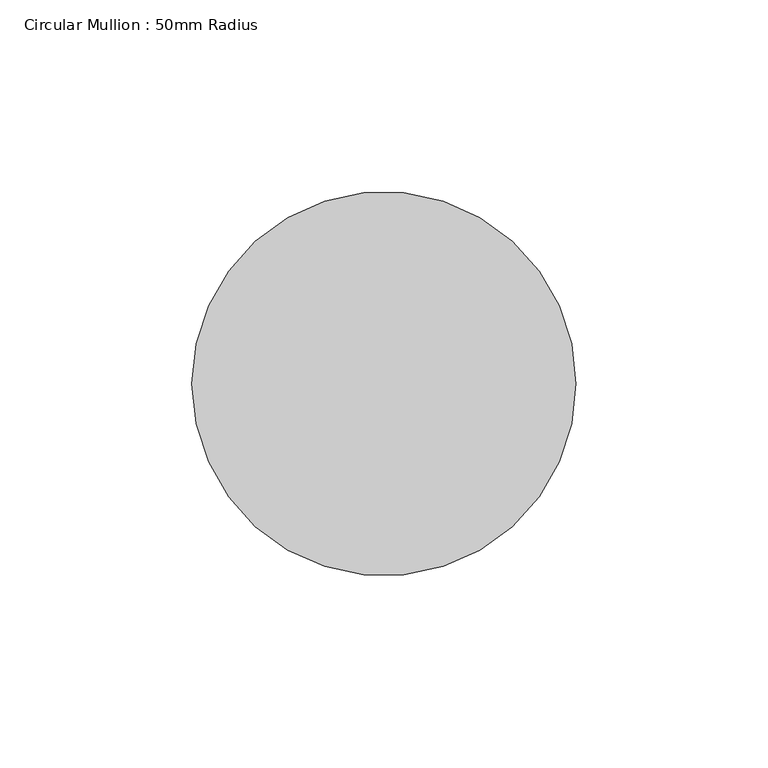
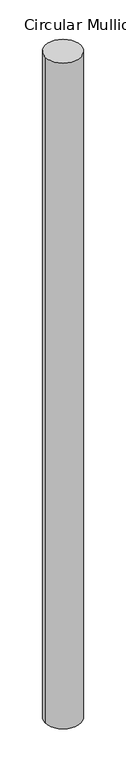
"""IFC4 building model written with IfcOpenShell, lengths in millimetres: member geometry, Circular Mullion : 50mm Radius."""

from ifc_helpers import new_model, si_unit, point, frame, frame_2d, origin, place, context, project, spatial, circle_curve, trimmed, segment, composite_curve, outline, extrude, source, transform, mapped, element, save


def circular_mullion_50mm_radius_29af998c(model_context):
    return source(origin(), model_context, "Body", "SweptSolid", [
        extrude(outline(composite_curve([segment(trimmed(circle_curve(frame_2d((-50.0, 0.0)), 50.0), [point((0.0, 0.0))], [point((-100.0, 0.0))], False, "CARTESIAN"), True, "CONTINUOUS"), segment(trimmed(circle_curve(frame_2d((-50.0, 0.0)), 50.0), [point((-100.0, 0.0))], [point((0.0, 0.0))], False, "CARTESIAN"), True, "CONTINUOUS")], self_intersect=False)), frame((0.0, 0.0, -1961.2253741), z_axis=(0.0, 0.0, 1.0), x_axis=(1.0, 0.0, 0.0)), (0.0, 0.0, 1.0), 1961.2253741),
    ])


if __name__ == "__main__":
    model = new_model("IFC4")
    model_context = context("Model", 3, world=origin())
    ifc_project = project(units=[si_unit("LENGTHUNIT", "METRE", prefix="MILLI")], contexts=[model_context])
    site = spatial("IfcSite", under=ifc_project)
    building = spatial("IfcBuilding", under=site)
    placement = place(None, origin())
    circular_mullion_50mm_radius_shape = circular_mullion_50mm_radius_29af998c(model_context)
    element("IfcMember", 1, ObjectType="Circular Mullion : 50mm Radius", at=placement, inside=building, context=model_context, shape_type="MappedRepresentation", body=[
        mapped(circular_mullion_50mm_radius_shape, transform((0.0, 0.0, 0.0), x_axis=(1.0, 0.0, 0.0), y_axis=(0.0, 1.0, 0.0), z_axis=(0.0, 0.0, 1.0))),
    ])
    save(model, "model.ifc")

# Revit data of these elements
# Type "Circular Mullion : 50mm Radius"
#   built-in parameter 1007350 = 0.164042 (stored number, unit not read)
# Element 1 (IfcMember, "Circular Mullion : 50mm Radius")
#   Materials on its faces: "Aluminium"
# Materials
#   "Aluminium": class "Metal", colour RGB 247 247 247, transparency 0, Description = "Aluminium 6061", Cost = 0
